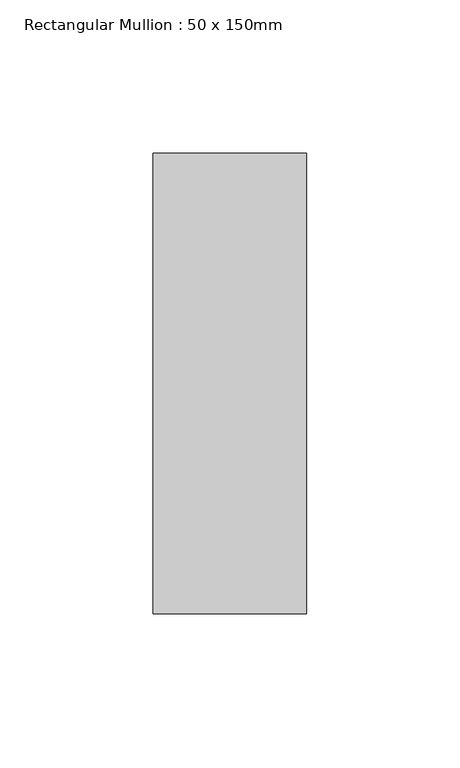
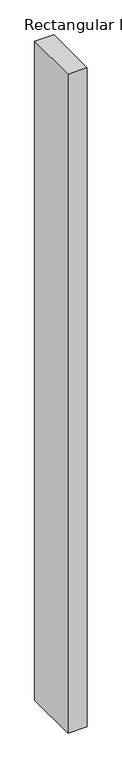
"""IFC4 building model written with IfcOpenShell, lengths in millimetres: member geometry, Rectangular Mullion : 50 x 150mm."""

from ifc_helpers import new_model, si_unit, frame, origin, place, context, project, spatial, polyline, outline, extrude, source, transform, mapped, element, save


def rectangular_mullion_50_x_150mm_dd1ee420(model_context):
    return source(origin(), model_context, "Body", "SweptSolid", [
        extrude(outline(polyline([(0.0, 75.0), (0.0, -75.0), (-50.0, -75.0), (-50.0, 75.0), (0.0, 75.0)])), frame((0.0, 0.0, -1811.1666669), z_axis=(0.0, 0.0, 1.0), x_axis=(1.0, 0.0, 0.0)), (0.0, 0.0, 1.0), 1811.1666669),
    ])


if __name__ == "__main__":
    model = new_model("IFC4")
    model_context = context("Model", 3, world=origin())
    ifc_project = project(units=[si_unit("LENGTHUNIT", "METRE", prefix="MILLI")], contexts=[model_context])
    site = spatial("IfcSite", under=ifc_project)
    building = spatial("IfcBuilding", under=site)
    placement = place(None, origin())
    rectangular_mullion_50_x_150mm_shape = rectangular_mullion_50_x_150mm_dd1ee420(model_context)
    element("IfcMember", 1, ObjectType="Rectangular Mullion : 50 x 150mm", at=placement, inside=building, context=model_context, shape_type="MappedRepresentation", body=[
        mapped(rectangular_mullion_50_x_150mm_shape, transform((0.0, 0.0, 0.0), x_axis=(1.0, 0.0, 0.0), y_axis=(0.0, 1.0, 0.0), z_axis=(0.0, 0.0, 1.0))),
    ])
    save(model, "model.ifc")

# Revit data of these elements
# Type "Rectangular Mullion : 50 x 150mm"
#   built-in parameter 1007304 = 0.492126 (stored number, unit not read)
#   built-in parameter 1007301 = 0.082021 (stored number, unit not read)
#   built-in parameter 1007300 = 0.082021 (stored number, unit not read)
# Element 1 (IfcMember, "Rectangular Mullion : 50 x 150mm")
#   Materials on its faces: "Metal - Aluminium"
# Materials
#   "Metal - Aluminium": class "Metal", colour RGB 247 247 247, transparency 0
